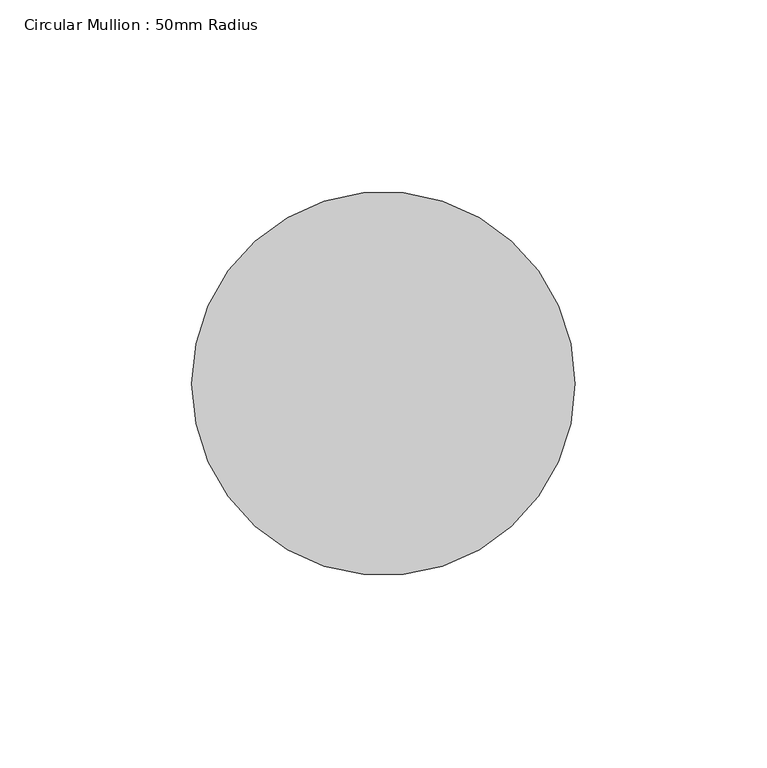
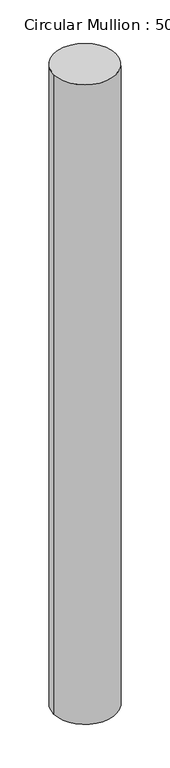
"""IFC4 building model written with IfcOpenShell, lengths in millimetres: member geometry, Circular Mullion : 50mm Radius."""

from ifc_helpers import new_model, si_unit, point, frame, origin, origin_2d, place, context, project, spatial, circle_curve, trimmed, segment, composite_curve, outline, extrude, source, transform, mapped, element, save


def circular_mullion_50mm_radius_111f5505(model_context):
    return source(origin(), model_context, "Body", "SweptSolid", [
        extrude(outline(composite_curve([segment(trimmed(circle_curve(origin_2d(), 50.0), [point((50.0, 0.0))], [point((-50.0, 0.0))], False, "CARTESIAN"), True, "CONTINUOUS"), segment(trimmed(circle_curve(origin_2d(), 50.0), [point((-50.0, 0.0))], [point((50.0, 0.0))], False, "CARTESIAN"), True, "CONTINUOUS")], self_intersect=False)), frame((0.0, 0.0, -1084.8681487), z_axis=(0.0, 0.0, 1.0), x_axis=(1.0, 0.0, 0.0)), (0.0, 0.0, 1.0), 1084.8681487),
    ])


if __name__ == "__main__":
    model = new_model("IFC4")
    model_context = context("Model", 3, world=origin())
    ifc_project = project(units=[si_unit("LENGTHUNIT", "METRE", prefix="MILLI")], contexts=[model_context])
    site = spatial("IfcSite", under=ifc_project)
    building = spatial("IfcBuilding", under=site)
    placement = place(None, origin())
    circular_mullion_50mm_radius_shape = circular_mullion_50mm_radius_111f5505(model_context)
    element("IfcMember", 1, ObjectType="Circular Mullion : 50mm Radius", at=placement, inside=building, context=model_context, shape_type="MappedRepresentation", body=[
        mapped(circular_mullion_50mm_radius_shape, transform((0.0, 0.0, 0.0), x_axis=(1.0, 0.0, 0.0), y_axis=(0.0, 1.0, 0.0), z_axis=(0.0, 0.0, 1.0))),
    ])
    save(model, "model.ifc")

# Revit data of these elements
# Type "Circular Mullion : 50mm Radius"
#   built-in parameter 1007350 = 0.164042 (stored number, unit not read)
# Element 1 (IfcMember, "Circular Mullion : 50mm Radius")
#   Materials on its faces: "Aluminium"
# Materials
#   "Aluminium": class "Metal", colour RGB 247 247 247, transparency 0, Description = "Aluminium 6061", Cost = 0
